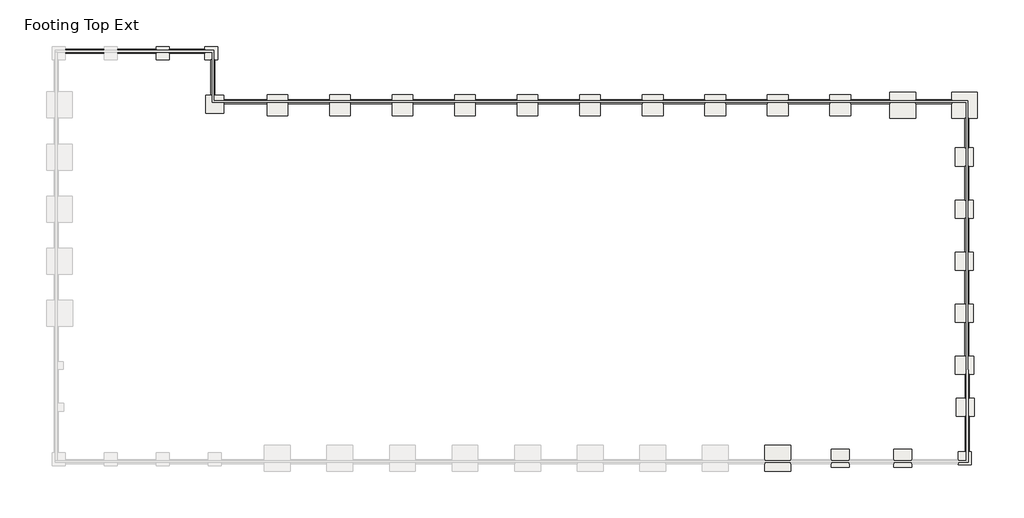
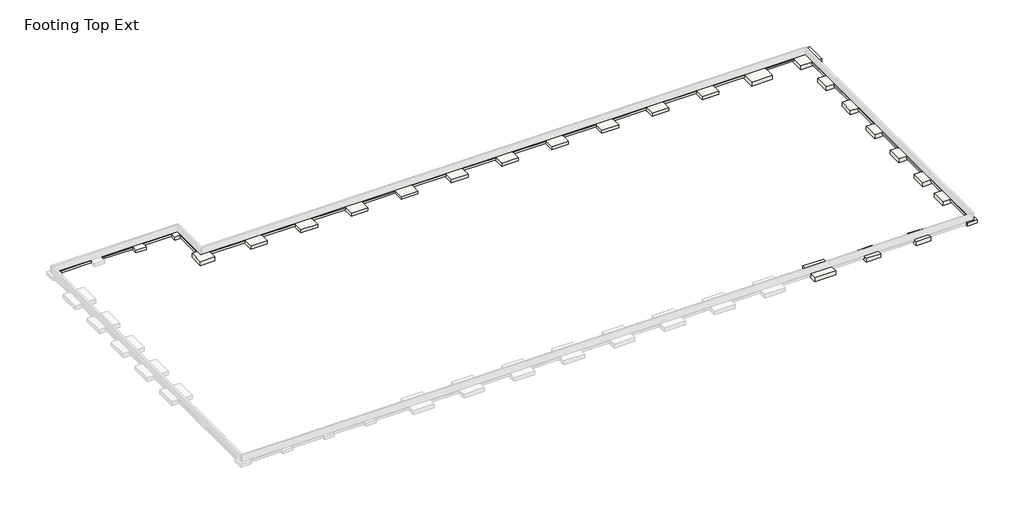
# One storey, part 2 of 2: 25 slabs, 5 footings.
"""IFC4 building model written with IfcOpenShell, lengths in millimetres."""

from ifc_helpers import new_model, si_unit, frame, origin, place, context, project, spatial, polyline, outline, extrude, faceted_brep, element, save

model = new_model("IFC4")

# Units and contexts
model_context = context("Model", 3, world=origin())
ifc_project = project(units=[si_unit("LENGTHUNIT", "METRE", prefix="MILLI")], contexts=[model_context])

# Site, building, storey
site = spatial("IfcSite", under=ifc_project)
building = spatial("IfcBuilding", under=site)
storey = spatial("IfcBuildingStorey", under=building, Name="Footing Top Ext", Elevation=-1066.8)

# Footings
placement = place(None, origin())
element("IfcFooting", 1, ObjectType="Bearing Footing - 18\" x 12\"", at=placement, inside=storey, context=model_context, shape_type="SweptSolid", body=[
    extrude(outline(polyline([(305655.7648264, -530975.6413841), (305655.7648264, -530518.4413841), (310230.9398264, -530518.4413841), (310230.9398264, -530975.6413841), (305655.7648264, -530975.6413841)])), frame((0.0, 0.0, -1371.6), z_axis=(0.0, 0.0, 1.0), x_axis=(1.0, 0.0, 0.0)), (0.0, 0.0, 1.0), 304.8),
    extrude(outline(polyline([(317882.6898264, -530975.6413841), (317882.6898264, -530518.4413841), (322051.4648264, -530518.4413841), (322051.4648264, -530975.6413841), (317882.6898264, -530975.6413841)])), frame((0.0, 0.0, -1371.6), z_axis=(0.0, 0.0, 1.0), x_axis=(1.0, 0.0, 0.0)), (0.0, 0.0, 1.0), 304.8),
    extrude(outline(polyline([(316358.6898264, -530518.4413841), (316358.6898264, -530975.6413841), (311754.9398264, -530975.6413841), (311754.9398264, -530518.4413841), (316358.6898264, -530518.4413841)])), frame((0.0, 0.0, -1371.6), z_axis=(0.0, 0.0, 1.0), x_axis=(1.0, 0.0, 0.0)), (0.0, 0.0, 1.0), 304.8),
])
element("IfcFooting", 2, ObjectType="Bearing Footing - 18\" x 12\"", at=placement, inside=storey, context=model_context, shape_type="SweptSolid", body=[
    extrude(outline(polyline([(322791.2398264, -531712.2413841), (323248.4398264, -531712.2413841), (323248.4398264, -535903.2413841), (322791.2398264, -535903.2413841), (322791.2398264, -531712.2413841)])), frame((0.0, 0.0, -1371.6), z_axis=(0.0, 0.0, 1.0), x_axis=(1.0, 0.0, 0.0)), (0.0, 0.0, 1.0), 304.8),
])
element("IfcFooting", 3, ObjectType="Bearing Footing - 18\" x 12\"", at=placement, inside=storey, context=model_context, shape_type="SweptSolid", body=[
    extrude(outline(polyline([(409862.4397781, -536430.2913841), (409862.4397781, -536887.4913841), (405658.7398264, -536887.4913841), (405658.7398264, -536430.2913841), (409862.4397781, -536430.2913841)])), frame((0.0, 0.0, -1371.6), z_axis=(0.0, 0.0, 1.0), x_axis=(1.0, 0.0, 0.0)), (0.0, 0.0, 1.0), 304.8),
    extrude(outline(polyline([(402610.7398264, -536430.2913841), (402610.7398264, -536887.4913841), (398000.6398264, -536887.4913841), (398000.6398264, -536430.2913841), (402610.7398264, -536430.2913841)])), frame((0.0, 0.0, -1371.6), z_axis=(0.0, 0.0, 1.0), x_axis=(1.0, 0.0, 0.0)), (0.0, 0.0, 1.0), 304.8),
    extrude(outline(polyline([(395562.2398264, -536430.2913841), (395562.2398264, -536887.4913841), (390647.3398264, -536887.4913841), (390647.3398264, -536430.2913841), (395562.2398264, -536430.2913841)])), frame((0.0, 0.0, -1371.6), z_axis=(0.0, 0.0, 1.0), x_axis=(1.0, 0.0, 0.0)), (0.0, 0.0, 1.0), 304.8),
    extrude(outline(polyline([(388208.9398264, -536430.2913841), (388208.9398264, -536887.4913841), (383294.0398264, -536887.4913841), (383294.0398264, -536430.2913841), (388208.9398264, -536430.2913841)])), frame((0.0, 0.0, -1371.6), z_axis=(0.0, 0.0, 1.0), x_axis=(1.0, 0.0, 0.0)), (0.0, 0.0, 1.0), 304.8),
    extrude(outline(polyline([(380855.6398264, -536430.2913841), (380855.6398264, -536887.4913841), (375940.7398264, -536887.4913841), (375940.7398264, -536430.2913841), (380855.6398264, -536430.2913841)])), frame((0.0, 0.0, -1371.6), z_axis=(0.0, 0.0, 1.0), x_axis=(1.0, 0.0, 0.0)), (0.0, 0.0, 1.0), 304.8),
    extrude(outline(polyline([(373502.3398264, -536430.2913841), (373502.3398264, -536887.4913841), (368587.4398264, -536887.4913841), (368587.4398264, -536430.2913841), (373502.3398264, -536430.2913841)])), frame((0.0, 0.0, -1371.6), z_axis=(0.0, 0.0, 1.0), x_axis=(1.0, 0.0, 0.0)), (0.0, 0.0, 1.0), 304.8),
    extrude(outline(polyline([(366149.0398264, -536430.2913841), (366149.0398264, -536887.4913841), (361234.1398264, -536887.4913841), (361234.1398264, -536430.2913841), (366149.0398264, -536430.2913841)])), frame((0.0, 0.0, -1371.6), z_axis=(0.0, 0.0, 1.0), x_axis=(1.0, 0.0, 0.0)), (0.0, 0.0, 1.0), 304.8),
    extrude(outline(polyline([(358795.7398264, -536430.2913841), (358795.7398264, -536887.4913841), (353880.8398264, -536887.4913841), (353880.8398264, -536430.2913841), (358795.7398264, -536430.2913841)])), frame((0.0, 0.0, -1371.6), z_axis=(0.0, 0.0, 1.0), x_axis=(1.0, 0.0, 0.0)), (0.0, 0.0, 1.0), 304.8),
    extrude(outline(polyline([(351442.4398264, -536430.2913841), (351442.4398264, -536887.4913841), (346527.5398264, -536887.4913841), (346527.5398264, -536430.2913841), (351442.4398264, -536430.2913841)])), frame((0.0, 0.0, -1371.6), z_axis=(0.0, 0.0, 1.0), x_axis=(1.0, 0.0, 0.0)), (0.0, 0.0, 1.0), 304.8),
    extrude(outline(polyline([(344089.1398264, -536430.2913841), (344089.1398264, -536887.4913841), (339174.2398264, -536887.4913841), (339174.2398264, -536430.2913841), (344089.1398264, -536430.2913841)])), frame((0.0, 0.0, -1371.6), z_axis=(0.0, 0.0, 1.0), x_axis=(1.0, 0.0, 0.0)), (0.0, 0.0, 1.0), 304.8),
    extrude(outline(polyline([(336735.8398264, -536430.2913841), (336735.8398264, -536887.4913841), (331820.9398264, -536887.4913841), (331820.9398264, -536430.2913841), (336735.8398264, -536430.2913841)])), frame((0.0, 0.0, -1371.6), z_axis=(0.0, 0.0, 1.0), x_axis=(1.0, 0.0, 0.0)), (0.0, 0.0, 1.0), 304.8),
    extrude(outline(polyline([(329382.5398264, -536430.2913841), (329382.5398264, -536887.4913841), (324289.8398264, -536887.4913841), (324289.8398264, -536430.2913841), (329382.5398264, -536430.2913841)])), frame((0.0, 0.0, -1371.6), z_axis=(0.0, 0.0, 1.0), x_axis=(1.0, 0.0, 0.0)), (0.0, 0.0, 1.0), 304.8),
])
element("IfcFooting", 4, ObjectType="Bearing Footing - 18\" x 12\"", at=placement, inside=storey, context=model_context, shape_type="SweptSolid", body=[
    extrude(outline(polyline([(411894.4398264, -560496.7913841), (411437.2398264, -560496.7913841), (411437.2398264, -556502.6413841), (411894.4398264, -556502.6413841), (411894.4398264, -560496.7913841)])), frame((0.0, 0.0, -1371.6), z_axis=(0.0, 0.0, 1.0), x_axis=(1.0, 0.0, 0.0)), (0.0, 0.0, 1.0), 304.8),
    extrude(outline(polyline([(411437.2398264, -562630.3913841), (411894.4398264, -562630.3913841), (411894.4398264, -566599.1414082), (411437.2398264, -566599.1414082), (411437.2398264, -562630.3913841)])), frame((0.0, 0.0, -1371.6), z_axis=(0.0, 0.0, 1.0), x_axis=(1.0, 0.0, 0.0)), (0.0, 0.0, 1.0), 304.8),
    extrude(outline(polyline([(411894.4398264, -554369.0413841), (411437.2398264, -554369.0413841), (411437.2398264, -550374.8913841), (411894.4398264, -550374.8913841), (411894.4398264, -554369.0413841)])), frame((0.0, 0.0, -1371.6), z_axis=(0.0, 0.0, 1.0), x_axis=(1.0, 0.0, 0.0)), (0.0, 0.0, 1.0), 304.8),
    extrude(outline(polyline([(411894.4398264, -548241.2913841), (411437.2398264, -548241.2913841), (411437.2398264, -544247.1413841), (411894.4398264, -544247.1413841), (411894.4398264, -548241.2913841)])), frame((0.0, 0.0, -1371.6), z_axis=(0.0, 0.0, 1.0), x_axis=(1.0, 0.0, 0.0)), (0.0, 0.0, 1.0), 304.8),
    extrude(outline(polyline([(411894.4398264, -542113.5413841), (411437.2398264, -542113.5413841), (411437.2398264, -538601.9913841), (411894.4398264, -538601.9913841), (411894.4398264, -542113.5413841)])), frame((0.0, 0.0, -1371.6), z_axis=(0.0, 0.0, 1.0), x_axis=(1.0, 0.0, 0.0)), (0.0, 0.0, 1.0), 304.8),
])
element("IfcFooting", 5, ObjectType="Bearing Footing - 18\" x 12\"", at=placement, inside=storey, context=model_context, shape_type="SweptSolid", body=[
    extrude(outline(polyline([(411932.5398264, -577835.4663841), (411475.3398264, -577835.4663841), (411475.3398264, -573660.3413841), (411932.5398264, -573660.3413841), (411932.5398264, -577835.4663841)])), frame((0.0, 0.0, -1371.6), z_axis=(0.0, 0.0, 1.0), x_axis=(1.0, 0.0, 0.0)), (0.0, 0.0, 1.0), 304.8),
    extrude(outline(polyline([(411932.5398264, -571526.7413841), (411475.3398264, -571526.7413841), (411475.3398264, -568732.7414082), (411932.5398264, -568732.7414082), (411932.5398264, -571526.7413841)])), frame((0.0, 0.0, -1371.6), z_axis=(0.0, 0.0, 1.0), x_axis=(1.0, 0.0, 0.0)), (0.0, 0.0, 1.0), 304.8),
])

# Slabs
element("IfcSlab", 6, ObjectType="Footing-Rectangular : F10", at=placement, inside=storey, context=model_context, shape_type="Brep", body=[
    faceted_brep([(390952.1398264, -577079.8163841, -1066.8), (387904.1398264, -577079.8163841, -1066.8), (387904.1398264, -578759.3913841, -1066.8), (387904.1398264, -579216.5913841, -1066.8), (387904.1398264, -580127.8163841, -1066.8), (390952.1398264, -580127.8163841, -1066.8), (390952.1398264, -579216.5913841, -1066.8), (390952.1398264, -578759.3913841, -1066.8), (390952.1398264, -577079.8163841, -1676.4), (390952.1398264, -580127.8163841, -1676.4), (387904.1398264, -580127.8163841, -1676.4), (387904.1398264, -577079.8163841, -1676.4)], [[[0, 1, 2, 3, 4, 5, 6, 7]], [[8, 9, 10, 11]], [[1, 0, 8, 11]], [[4, 3, 2, 1, 11, 10]], [[5, 4, 10, 9]], [[0, 7, 6, 5, 9, 8]]]),
])
element("IfcSlab", 7, ObjectType="Footing-Rectangular : F10", at=placement, inside=storey, context=model_context, shape_type="Brep", body=[
    faceted_brep([(409862.4397781, -535553.9913841, -1066.8), (409862.4397781, -536430.2913841, -1066.8), (409862.4397781, -536887.4913841, -1066.8), (409862.4397781, -538601.9913841, -1066.8), (411437.2398264, -538601.9913841, -1066.8), (411894.4398264, -538601.9913841, -1066.8), (412910.4397781, -538601.9913841, -1066.8), (412910.4397781, -535553.9913841, -1066.8), (409862.4397781, -535553.9913841, -1676.4), (412910.4397781, -535553.9913841, -1676.4), (412910.4397781, -538601.9913841, -1676.4), (409862.4397781, -538601.9913841, -1676.4)], [[[0, 1, 2, 3, 4, 5, 6, 7]], [[8, 9, 10, 11]], [[3, 2, 1, 0, 8, 11]], [[6, 5, 4, 3, 11, 10]], [[7, 6, 10, 9]], [[0, 7, 9, 8]]]),
])
element("IfcSlab", 8, ObjectType="Footing-Rectangular : F10", at=placement, inside=storey, context=model_context, shape_type="Brep", body=[
    faceted_brep([(402610.7398264, -535553.9913841, -1066.8), (402610.7398264, -536430.2913841, -1066.8), (402610.7398264, -536887.4913841, -1066.8), (402610.7398264, -538601.9913841, -1066.8), (405658.7398264, -538601.9913841, -1066.8), (405658.7398264, -536887.4913841, -1066.8), (405658.7398264, -536430.2913841, -1066.8), (405658.7398264, -535553.9913841, -1066.8), (402610.7398264, -535553.9913841, -1676.4), (405658.7398264, -535553.9913841, -1676.4), (405658.7398264, -538601.9913841, -1676.4), (402610.7398264, -538601.9913841, -1676.4)], [[[0, 1, 2, 3, 4, 5, 6, 7]], [[8, 9, 10, 11]], [[3, 2, 1, 0, 8, 11]], [[4, 3, 11, 10]], [[7, 6, 5, 4, 10, 9]], [[0, 7, 9, 8]]]),
])
element("IfcSlab", 9, ObjectType="Footing-Rectangular : F5", at=placement, inside=storey, context=model_context, shape_type="Brep", body=[
    faceted_brep([(317882.6898264, -530191.4163841, -1066.8), (316358.6898264, -530191.4163841, -1066.8), (316358.6898264, -530518.4413841, -1066.8), (316358.6898264, -530975.6413841, -1066.8), (316358.6898264, -531715.4163841, -1066.8), (317882.6898264, -531715.4163841, -1066.8), (317882.6898264, -530975.6413841, -1066.8), (317882.6898264, -530518.4413841, -1066.8), (317882.6898264, -530191.4163841, -1524.0), (317882.6898264, -531715.4163841, -1524.0), (316358.6898264, -531715.4163841, -1524.0), (316358.6898264, -530191.4163841, -1524.0)], [[[0, 1, 2, 3, 4, 5, 6, 7]], [[8, 9, 10, 11]], [[1, 0, 8, 11]], [[4, 3, 2, 1, 11, 10]], [[5, 4, 10, 9]], [[0, 7, 6, 5, 9, 8]]]),
])
element("IfcSlab", 10, ObjectType="Footing-Rectangular : F5", at=placement, inside=storey, context=model_context, shape_type="Brep", body=[
    faceted_brep([(323575.4648264, -530188.2413841, -1066.8), (322051.4648264, -530188.2413841, -1066.8), (322051.4648264, -530518.4413841, -1066.8), (322051.4648264, -530975.6413841, -1066.8), (322051.4648264, -531712.2413841, -1066.8), (322791.2398264, -531712.2413841, -1066.8), (323248.4398264, -531712.2413841, -1066.8), (323575.4648264, -531712.2413841, -1066.8), (323575.4648264, -530188.2413841, -1524.0), (323575.4648264, -531712.2413841, -1524.0), (322051.4648264, -531712.2413841, -1524.0), (322051.4648264, -530188.2413841, -1524.0)], [[[0, 1, 2, 3, 4, 5, 6, 7]], [[8, 9, 10, 11]], [[1, 0, 8, 11]], [[4, 3, 2, 1, 11, 10]], [[7, 6, 5, 4, 10, 9]], [[0, 7, 9, 8]]]),
])
element("IfcSlab", 11, ObjectType="Footing-Rectangular : F5", at=placement, inside=storey, context=model_context, shape_type="Brep", body=[
    faceted_brep([(412199.2398264, -577835.4663841, -1066.8), (411932.5398264, -577835.4663841, -1066.8), (411475.3398264, -577835.4663841, -1066.8), (410675.2398264, -577835.4663841, -1066.8), (410675.2398264, -578759.3913841, -1066.8), (410675.2398264, -579216.5913841, -1066.8), (410675.2398264, -579359.4663841, -1066.8), (412199.2398264, -579359.4663841, -1066.8), (412199.2398264, -577835.4663841, -1524.0), (412199.2398264, -579359.4663841, -1524.0), (410675.2398264, -579359.4663841, -1524.0), (410675.2398264, -577835.4663841, -1524.0)], [[[0, 1, 2, 3, 4, 5, 6, 7]], [[8, 9, 10, 11]], [[3, 2, 1, 0, 8, 11]], [[6, 5, 4, 3, 11, 10]], [[7, 6, 10, 9]], [[0, 7, 9, 8]]]),
])
element("IfcSlab", 12, ObjectType="Footing-Rectangular : F7", at=placement, inside=storey, context=model_context, shape_type="Brep", body=[
    faceted_brep([(397848.2398264, -577530.6663841, -1066.8), (395714.6398264, -577530.6663841, -1066.8), (395714.6398264, -578759.3913841, -1066.8), (395714.6398264, -579216.5913841, -1066.8), (395714.6398264, -579664.2663841, -1066.8), (397848.2398264, -579664.2663841, -1066.8), (397848.2398264, -579216.5913841, -1066.8), (397848.2398264, -578759.3913841, -1066.8), (397848.2398264, -577530.6663841, -1676.4), (397848.2398264, -579664.2663841, -1676.4), (395714.6398264, -579664.2663841, -1676.4), (395714.6398264, -577530.6663841, -1676.4)], [[[0, 1, 2, 3, 4, 5, 6, 7]], [[8, 9, 10, 11]], [[1, 0, 8, 11]], [[4, 3, 2, 1, 11, 10]], [[5, 4, 10, 9]], [[0, 7, 6, 5, 9, 8]]]),
])
element("IfcSlab", 13, ObjectType="Footing-Rectangular : F7", at=placement, inside=storey, context=model_context, shape_type="Brep", body=[
    faceted_brep([(405201.5398264, -577530.6663841, -1066.8), (403067.9398264, -577530.6663841, -1066.8), (403067.9398264, -578759.3913841, -1066.8), (403067.9398264, -579216.5913841, -1066.8), (403067.9398264, -579664.2663841, -1066.8), (405201.5398264, -579664.2663841, -1066.8), (405201.5398264, -579216.5913841, -1066.8), (405201.5398264, -578759.3913841, -1066.8), (405201.5398264, -577530.6663841, -1676.4), (405201.5398264, -579664.2663841, -1676.4), (403067.9398264, -579664.2663841, -1676.4), (403067.9398264, -577530.6663841, -1676.4)], [[[0, 1, 2, 3, 4, 5, 6, 7]], [[8, 9, 10, 11]], [[1, 0, 8, 11]], [[4, 3, 2, 1, 11, 10]], [[5, 4, 10, 9]], [[0, 7, 6, 5, 9, 8]]]),
])
element("IfcSlab", 14, ObjectType="Footing-Rectangular : F7", at=placement, inside=storey, context=model_context, shape_type="Brep", body=[
    faceted_brep([(412526.2648264, -571526.7413841, -1066.8), (411932.5398264, -571526.7413841, -1066.8), (411475.3398264, -571526.7413841, -1066.8), (410392.6648264, -571526.7413841, -1066.8), (410392.6648264, -573660.3413841, -1066.8), (411475.3398264, -573660.3413841, -1066.8), (411932.5398264, -573660.3413841, -1066.8), (412526.2648264, -573660.3413841, -1066.8), (412526.2648264, -571526.7413841, -1676.4), (412526.2648264, -573660.3413841, -1676.4), (410392.6648264, -573660.3413841, -1676.4), (410392.6648264, -571526.7413841, -1676.4)], [[[0, 1, 2, 3, 4, 5, 6, 7]], [[8, 9, 10, 11]], [[3, 2, 1, 0, 8, 11]], [[4, 3, 11, 10]], [[7, 6, 5, 4, 10, 9]], [[0, 7, 9, 8]]]),
])
element("IfcSlab", 15, ObjectType="Footing-Rectangular : F7", at=placement, inside=storey, context=model_context, shape_type="Brep", body=[
    faceted_brep([(410319.6398264, -566599.1414082, -1066.8), (410319.6398264, -568732.7414082, -1066.8), (411475.3398264, -568732.7414082, -1066.8), (411932.5398264, -568732.7414082, -1066.8), (412453.2398264, -568732.7414082, -1066.8), (412453.2398264, -566599.1414082, -1066.8), (411894.4398264, -566599.1414082, -1066.8), (411437.2398264, -566599.1414082, -1066.8), (410319.6398264, -566599.1414082, -1676.4), (412453.2398264, -566599.1414082, -1676.4), (412453.2398264, -568732.7414082, -1676.4), (410319.6398264, -568732.7414082, -1676.4)], [[[0, 1, 2, 3, 4, 5, 6, 7]], [[8, 9, 10, 11]], [[1, 0, 8, 11]], [[4, 3, 2, 1, 11, 10]], [[5, 4, 10, 9]], [[0, 7, 6, 5, 9, 8]]]),
])
element("IfcSlab", 16, ObjectType="Footing-Rectangular : F7", at=placement, inside=storey, context=model_context, shape_type="Brep", body=[
    faceted_brep([(412443.7148264, -560496.7913841, -1066.8), (411894.4398264, -560496.7913841, -1066.8), (411437.2398264, -560496.7913841, -1066.8), (410310.1148264, -560496.7913841, -1066.8), (410310.1148264, -562630.3913841, -1066.8), (411437.2398264, -562630.3913841, -1066.8), (411894.4398264, -562630.3913841, -1066.8), (412443.7148264, -562630.3913841, -1066.8), (412443.7148264, -560496.7913841, -1676.4), (412443.7148264, -562630.3913841, -1676.4), (410310.1148264, -562630.3913841, -1676.4), (410310.1148264, -560496.7913841, -1676.4)], [[[0, 1, 2, 3, 4, 5, 6, 7]], [[8, 9, 10, 11]], [[3, 2, 1, 0, 8, 11]], [[4, 3, 11, 10]], [[7, 6, 5, 4, 10, 9]], [[0, 7, 9, 8]]]),
])
element("IfcSlab", 17, ObjectType="Footing-Rectangular : F7", at=placement, inside=storey, context=model_context, shape_type="Brep", body=[
    faceted_brep([(412443.7148264, -554369.0413841, -1066.8), (411894.4398264, -554369.0413841, -1066.8), (411437.2398264, -554369.0413841, -1066.8), (410310.1148264, -554369.0413841, -1066.8), (410310.1148264, -556502.6413841, -1066.8), (411437.2398264, -556502.6413841, -1066.8), (411894.4398264, -556502.6413841, -1066.8), (412443.7148264, -556502.6413841, -1066.8), (412443.7148264, -554369.0413841, -1676.4), (412443.7148264, -556502.6413841, -1676.4), (410310.1148264, -556502.6413841, -1676.4), (410310.1148264, -554369.0413841, -1676.4)], [[[0, 1, 2, 3, 4, 5, 6, 7]], [[8, 9, 10, 11]], [[3, 2, 1, 0, 8, 11]], [[4, 3, 11, 10]], [[7, 6, 5, 4, 10, 9]], [[0, 7, 9, 8]]]),
])
element("IfcSlab", 18, ObjectType="Footing-Rectangular : F7", at=placement, inside=storey, context=model_context, shape_type="Brep", body=[
    faceted_brep([(412443.7148264, -548241.2913841, -1066.8), (411894.4398264, -548241.2913841, -1066.8), (411437.2398264, -548241.2913841, -1066.8), (410310.1148264, -548241.2913841, -1066.8), (410310.1148264, -550374.8913841, -1066.8), (411437.2398264, -550374.8913841, -1066.8), (411894.4398264, -550374.8913841, -1066.8), (412443.7148264, -550374.8913841, -1066.8), (412443.7148264, -548241.2913841, -1676.4), (412443.7148264, -550374.8913841, -1676.4), (410310.1148264, -550374.8913841, -1676.4), (410310.1148264, -548241.2913841, -1676.4)], [[[0, 1, 2, 3, 4, 5, 6, 7]], [[8, 9, 10, 11]], [[3, 2, 1, 0, 8, 11]], [[4, 3, 11, 10]], [[7, 6, 5, 4, 10, 9]], [[0, 7, 9, 8]]]),
])
element("IfcSlab", 19, ObjectType="Footing-Rectangular : F7", at=placement, inside=storey, context=model_context, shape_type="Brep", body=[
    faceted_brep([(412443.7148264, -542113.5413841, -1066.8), (411894.4398264, -542113.5413841, -1066.8), (411437.2398264, -542113.5413841, -1066.8), (410310.1148264, -542113.5413841, -1066.8), (410310.1148264, -544247.1413841, -1066.8), (411437.2398264, -544247.1413841, -1066.8), (411894.4398264, -544247.1413841, -1066.8), (412443.7148264, -544247.1413841, -1066.8), (412443.7148264, -542113.5413841, -1676.4), (412443.7148264, -544247.1413841, -1676.4), (410310.1148264, -544247.1413841, -1676.4), (410310.1148264, -542113.5413841, -1676.4)], [[[0, 1, 2, 3, 4, 5, 6, 7]], [[8, 9, 10, 11]], [[3, 2, 1, 0, 8, 11]], [[4, 3, 11, 10]], [[7, 6, 5, 4, 10, 9]], [[0, 7, 9, 8]]]),
])
element("IfcSlab", 20, ObjectType="Footing-Rectangular : F7", at=placement, inside=storey, context=model_context, shape_type="Brep", body=[
    faceted_brep([(322156.2398264, -535903.2413841, -1066.8), (322156.2398264, -538036.8413841, -1066.8), (324289.8398264, -538036.8413841, -1066.8), (324289.8398264, -536887.4913841, -1066.8), (324289.8398264, -536430.2913841, -1066.8), (324289.8398264, -535903.2413841, -1066.8), (323248.4398264, -535903.2413841, -1066.8), (322791.2398264, -535903.2413841, -1066.8), (322156.2398264, -535903.2413841, -1676.4), (324289.8398264, -535903.2413841, -1676.4), (324289.8398264, -538036.8413841, -1676.4), (322156.2398264, -538036.8413841, -1676.4)], [[[0, 1, 2, 3, 4, 5, 6, 7]], [[8, 9, 10, 11]], [[1, 0, 8, 11]], [[2, 1, 11, 10]], [[5, 4, 3, 2, 10, 9]], [[0, 7, 6, 5, 9, 8]]]),
])
element("IfcSlab", 21, ObjectType="Footing-Rectangular : F8", at=placement, inside=storey, context=model_context, shape_type="Brep", body=[
    faceted_brep([(395562.2398264, -535858.7913841, -1066.8), (395562.2398264, -536430.2913841, -1066.8), (395562.2398264, -536887.4913841, -1066.8), (395562.2398264, -538297.1913841, -1066.8), (398000.6398264, -538297.1913841, -1066.8), (398000.6398264, -536887.4913841, -1066.8), (398000.6398264, -536430.2913841, -1066.8), (398000.6398264, -535858.7913841, -1066.8), (395562.2398264, -535858.7913841, -1524.0), (398000.6398264, -535858.7913841, -1524.0), (398000.6398264, -538297.1913841, -1524.0), (395562.2398264, -538297.1913841, -1524.0)], [[[0, 1, 2, 3, 4, 5, 6, 7]], [[8, 9, 10, 11]], [[3, 2, 1, 0, 8, 11]], [[4, 3, 11, 10]], [[7, 6, 5, 4, 10, 9]], [[0, 7, 9, 8]]]),
])
element("IfcSlab", 22, ObjectType="Footing-Rectangular : F8", at=placement, inside=storey, context=model_context, shape_type="Brep", body=[
    faceted_brep([(388208.9398264, -535858.7913841, -1066.8), (388208.9398264, -536430.2913841, -1066.8), (388208.9398264, -536887.4913841, -1066.8), (388208.9398264, -538297.1913841, -1066.8), (390647.3398264, -538297.1913841, -1066.8), (390647.3398264, -536887.4913841, -1066.8), (390647.3398264, -536430.2913841, -1066.8), (390647.3398264, -535858.7913841, -1066.8), (388208.9398264, -535858.7913841, -1524.0), (390647.3398264, -535858.7913841, -1524.0), (390647.3398264, -538297.1913841, -1524.0), (388208.9398264, -538297.1913841, -1524.0)], [[[0, 1, 2, 3, 4, 5, 6, 7]], [[8, 9, 10, 11]], [[3, 2, 1, 0, 8, 11]], [[4, 3, 11, 10]], [[7, 6, 5, 4, 10, 9]], [[0, 7, 9, 8]]]),
])
element("IfcSlab", 23, ObjectType="Footing-Rectangular : F8", at=placement, inside=storey, context=model_context, shape_type="Brep", body=[
    faceted_brep([(380855.6398264, -535858.7913841, -1066.8), (380855.6398264, -536430.2913841, -1066.8), (380855.6398264, -536887.4913841, -1066.8), (380855.6398264, -538297.1913841, -1066.8), (383294.0398264, -538297.1913841, -1066.8), (383294.0398264, -536887.4913841, -1066.8), (383294.0398264, -536430.2913841, -1066.8), (383294.0398264, -535858.7913841, -1066.8), (380855.6398264, -535858.7913841, -1524.0), (383294.0398264, -535858.7913841, -1524.0), (383294.0398264, -538297.1913841, -1524.0), (380855.6398264, -538297.1913841, -1524.0)], [[[0, 1, 2, 3, 4, 5, 6, 7]], [[8, 9, 10, 11]], [[3, 2, 1, 0, 8, 11]], [[4, 3, 11, 10]], [[7, 6, 5, 4, 10, 9]], [[0, 7, 9, 8]]]),
])
element("IfcSlab", 24, ObjectType="Footing-Rectangular : F8", at=placement, inside=storey, context=model_context, shape_type="Brep", body=[
    faceted_brep([(373502.3398264, -535858.7913841, -1066.8), (373502.3398264, -536430.2913841, -1066.8), (373502.3398264, -536887.4913841, -1066.8), (373502.3398264, -538297.1913841, -1066.8), (375940.7398264, -538297.1913841, -1066.8), (375940.7398264, -536887.4913841, -1066.8), (375940.7398264, -536430.2913841, -1066.8), (375940.7398264, -535858.7913841, -1066.8), (373502.3398264, -535858.7913841, -1524.0), (375940.7398264, -535858.7913841, -1524.0), (375940.7398264, -538297.1913841, -1524.0), (373502.3398264, -538297.1913841, -1524.0)], [[[0, 1, 2, 3, 4, 5, 6, 7]], [[8, 9, 10, 11]], [[3, 2, 1, 0, 8, 11]], [[4, 3, 11, 10]], [[7, 6, 5, 4, 10, 9]], [[0, 7, 9, 8]]]),
])
element("IfcSlab", 25, ObjectType="Footing-Rectangular : F8", at=placement, inside=storey, context=model_context, shape_type="Brep", body=[
    faceted_brep([(366149.0398264, -535858.7913841, -1066.8), (366149.0398264, -536430.2913841, -1066.8), (366149.0398264, -536887.4913841, -1066.8), (366149.0398264, -538297.1913841, -1066.8), (368587.4398264, -538297.1913841, -1066.8), (368587.4398264, -536887.4913841, -1066.8), (368587.4398264, -536430.2913841, -1066.8), (368587.4398264, -535858.7913841, -1066.8), (366149.0398264, -535858.7913841, -1524.0), (368587.4398264, -535858.7913841, -1524.0), (368587.4398264, -538297.1913841, -1524.0), (366149.0398264, -538297.1913841, -1524.0)], [[[0, 1, 2, 3, 4, 5, 6, 7]], [[8, 9, 10, 11]], [[3, 2, 1, 0, 8, 11]], [[4, 3, 11, 10]], [[7, 6, 5, 4, 10, 9]], [[0, 7, 9, 8]]]),
])
element("IfcSlab", 26, ObjectType="Footing-Rectangular : F8", at=placement, inside=storey, context=model_context, shape_type="Brep", body=[
    faceted_brep([(358795.7398264, -535858.7913841, -1066.8), (358795.7398264, -536430.2913841, -1066.8), (358795.7398264, -536887.4913841, -1066.8), (358795.7398264, -538297.1913841, -1066.8), (361234.1398264, -538297.1913841, -1066.8), (361234.1398264, -536887.4913841, -1066.8), (361234.1398264, -536430.2913841, -1066.8), (361234.1398264, -535858.7913841, -1066.8), (358795.7398264, -535858.7913841, -1524.0), (361234.1398264, -535858.7913841, -1524.0), (361234.1398264, -538297.1913841, -1524.0), (358795.7398264, -538297.1913841, -1524.0)], [[[0, 1, 2, 3, 4, 5, 6, 7]], [[8, 9, 10, 11]], [[3, 2, 1, 0, 8, 11]], [[4, 3, 11, 10]], [[7, 6, 5, 4, 10, 9]], [[0, 7, 9, 8]]]),
])
element("IfcSlab", 27, ObjectType="Footing-Rectangular : F8", at=placement, inside=storey, context=model_context, shape_type="Brep", body=[
    faceted_brep([(351442.4398264, -535858.7913841, -1066.8), (351442.4398264, -536430.2913841, -1066.8), (351442.4398264, -536887.4913841, -1066.8), (351442.4398264, -538297.1913841, -1066.8), (353880.8398264, -538297.1913841, -1066.8), (353880.8398264, -536887.4913841, -1066.8), (353880.8398264, -536430.2913841, -1066.8), (353880.8398264, -535858.7913841, -1066.8), (351442.4398264, -535858.7913841, -1524.0), (353880.8398264, -535858.7913841, -1524.0), (353880.8398264, -538297.1913841, -1524.0), (351442.4398264, -538297.1913841, -1524.0)], [[[0, 1, 2, 3, 4, 5, 6, 7]], [[8, 9, 10, 11]], [[3, 2, 1, 0, 8, 11]], [[4, 3, 11, 10]], [[7, 6, 5, 4, 10, 9]], [[0, 7, 9, 8]]]),
])
element("IfcSlab", 28, ObjectType="Footing-Rectangular : F8", at=placement, inside=storey, context=model_context, shape_type="Brep", body=[
    faceted_brep([(344089.1398264, -535858.7913841, -1066.8), (344089.1398264, -536430.2913841, -1066.8), (344089.1398264, -536887.4913841, -1066.8), (344089.1398264, -538297.1913841, -1066.8), (346527.5398264, -538297.1913841, -1066.8), (346527.5398264, -536887.4913841, -1066.8), (346527.5398264, -536430.2913841, -1066.8), (346527.5398264, -535858.7913841, -1066.8), (344089.1398264, -535858.7913841, -1524.0), (346527.5398264, -535858.7913841, -1524.0), (346527.5398264, -538297.1913841, -1524.0), (344089.1398264, -538297.1913841, -1524.0)], [[[0, 1, 2, 3, 4, 5, 6, 7]], [[8, 9, 10, 11]], [[3, 2, 1, 0, 8, 11]], [[4, 3, 11, 10]], [[7, 6, 5, 4, 10, 9]], [[0, 7, 9, 8]]]),
])
element("IfcSlab", 29, ObjectType="Footing-Rectangular : F8", at=placement, inside=storey, context=model_context, shape_type="Brep", body=[
    faceted_brep([(336735.8398264, -535858.7913841, -1066.8), (336735.8398264, -536430.2913841, -1066.8), (336735.8398264, -536887.4913841, -1066.8), (336735.8398264, -538297.1913841, -1066.8), (339174.2398264, -538297.1913841, -1066.8), (339174.2398264, -536887.4913841, -1066.8), (339174.2398264, -536430.2913841, -1066.8), (339174.2398264, -535858.7913841, -1066.8), (336735.8398264, -535858.7913841, -1524.0), (339174.2398264, -535858.7913841, -1524.0), (339174.2398264, -538297.1913841, -1524.0), (336735.8398264, -538297.1913841, -1524.0)], [[[0, 1, 2, 3, 4, 5, 6, 7]], [[8, 9, 10, 11]], [[3, 2, 1, 0, 8, 11]], [[4, 3, 11, 10]], [[7, 6, 5, 4, 10, 9]], [[0, 7, 9, 8]]]),
])
element("IfcSlab", 30, ObjectType="Footing-Rectangular : F8", at=placement, inside=storey, context=model_context, shape_type="Brep", body=[
    faceted_brep([(329382.5398264, -535858.7913841, -1066.8), (329382.5398264, -536430.2913841, -1066.8), (329382.5398264, -536887.4913841, -1066.8), (329382.5398264, -538297.1913841, -1066.8), (331820.9398264, -538297.1913841, -1066.8), (331820.9398264, -536887.4913841, -1066.8), (331820.9398264, -536430.2913841, -1066.8), (331820.9398264, -535858.7913841, -1066.8), (329382.5398264, -535858.7913841, -1524.0), (331820.9398264, -535858.7913841, -1524.0), (331820.9398264, -538297.1913841, -1524.0), (329382.5398264, -538297.1913841, -1524.0)], [[[0, 1, 2, 3, 4, 5, 6, 7]], [[8, 9, 10, 11]], [[3, 2, 1, 0, 8, 11]], [[4, 3, 11, 10]], [[7, 6, 5, 4, 10, 9]], [[0, 7, 9, 8]]]),
])

save(model, "model.ifc")

# Revit data of these elements
# Type "Bearing Footing - 18\" x 12\""
#   Assembly Code = "A1010110"
# Type "Footing-Rectangular : F10"
#   Assembly Code = "A1010100"
#   Width = 10' - 0"
#   Length = 10' - 0"
#   Thickness = 2' - 0"
#   Structural Material [instance default] = Concrete, Cast-in-Place gray
# Type "Footing-Rectangular : F5"
#   Assembly Code = "A1010100"
#   Width = 5' - 0"
#   Length = 5' - 0"
#   Thickness = 1' - 6"
#   Structural Material [instance default] = Concrete, Cast-in-Place gray
# Type "Footing-Rectangular : F7"
#   Assembly Code = "A1010100"
#   Width = 7' - 0"
#   Length = 7' - 0"
#   Thickness = 2' - 0"
#   Structural Material [instance default] = Concrete, Cast-in-Place gray
# Type "Footing-Rectangular : F8"
#   Assembly Code = "A1010100"
#   Width = 8' - 0"
#   Length = 8' - 0"
#   Thickness = 1' - 6"
#   Structural Material [instance default] = Concrete, Cast-in-Place gray
# Elements 1, 2, 3, 4, 5 (IfcFooting, "Bearing Footing - 18\" x 12\"")
#   Phase Created = New Construction
#   Materials on its faces: "Concrete, Cast-in-Place gray"
# Elements 6, 7, 8 (IfcSlab, "Footing-Rectangular : F10")
#   Comments = ""
#   Structural Material = Concrete, Cast-in-Place gray
#   Phase Created = New Construction
#   Materials on its faces: "Concrete, Cast-in-Place gray"
# Elements 9, 10, 11 (IfcSlab, "Footing-Rectangular : F5")
#   Comments = ""
#   Structural Material = Concrete, Cast-in-Place gray
#   Phase Created = New Construction
#   Materials on its faces: "Concrete, Cast-in-Place gray"
# Elements 12, 13, 14, 15, 16, 17, 18, 19, 20 (IfcSlab, "Footing-Rectangular : F7")
#   Comments = ""
#   Structural Material = Concrete, Cast-in-Place gray
#   Phase Created = New Construction
#   Materials on its faces: "Concrete, Cast-in-Place gray"
# Elements 21, 22, 23, 24, 25, 26, 27, 28, 29, 30 (IfcSlab, "Footing-Rectangular : F8")
#   Comments = ""
#   Structural Material = Concrete, Cast-in-Place gray
#   Phase Created = New Construction
#   Materials on its faces: "Concrete, Cast-in-Place gray"
# Materials
#   "Concrete, Cast-in-Place gray": class "Concrete", colour RGB 192 192 192, transparency 0, Description = "Cast-in-place concrete", Cost = 0
